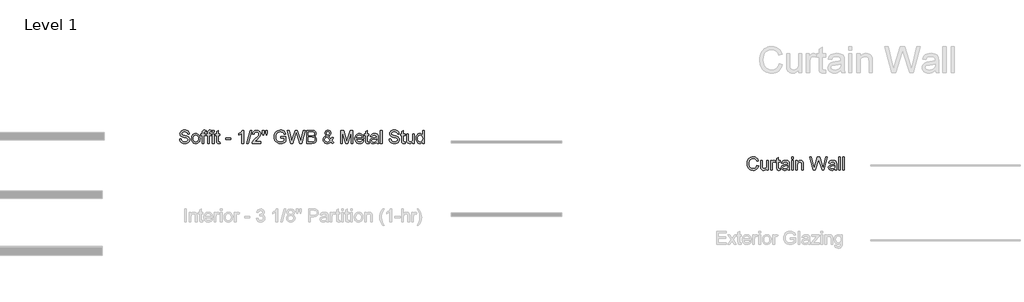
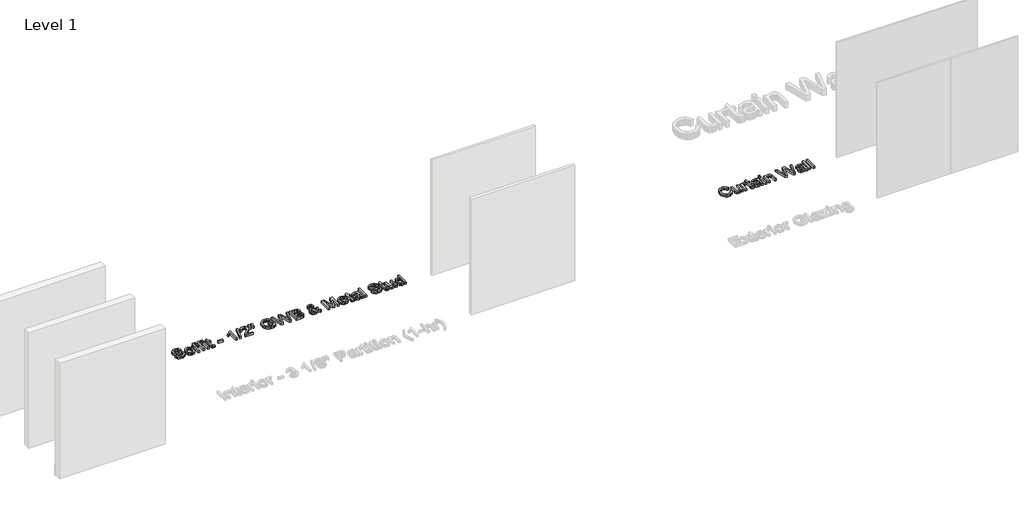
# One storey, part 40 of 42: 2 proxies.
"""IFC4 building model written with IfcOpenShell, lengths in millimetres."""

from ifc_helpers import new_model, si_unit, origin, origin_with_axes, place, context, project, spatial, polyline, outline, extrude, element, save

model = new_model("IFC4")

# Units and contexts
model_context = context("Model", 3, world=origin())
ifc_project = project(units=[si_unit("LENGTHUNIT", "METRE", prefix="MILLI")], contexts=[model_context])

# Site, building, storey
site = spatial("IfcSite", under=ifc_project)
building = spatial("IfcBuilding", under=site)
storey = spatial("IfcBuildingStorey", under=building, Name="Level 1", Elevation=0.0)

# Proxies
placement = place(None, origin())
element("IfcBuildingElementProxy", 1, Name="8\" Arial", ObjectType="8\" Arial", at=placement, inside=storey, context=model_context, shape_type="SweptSolid", body=[
    extrude(outline(polyline([(5120.6223042, 17413.5110871), (5158.693191, 17413.5110871), (5163.0616765, 17392.3843474), (5170.9621291, 17375.4030217), (5183.2868351, 17361.9257791), (5200.928081, 17351.3112887), (5222.4916692, 17344.423953), (5246.5834022, 17342.1281744), (5267.7937937, 17343.866274), (5286.3645046, 17349.0805727), (5301.4125431, 17357.3342219), (5312.0549174, 17368.1903732), (5318.3845741, 17380.654499), (5320.4944597, 17393.7320717), (5318.9143692, 17406.4750369), (5314.1740976, 17417.4891973), (5304.5448402, 17426.8860885), (5288.2977918, 17434.7772465), (5232.8644987, 17449.3140792), (5196.4759436, 17458.934042), (5173.1928451, 17468.0892724), (5154.2410536, 17480.8973002), (5140.8102842, 17496.4193658), (5132.8075905, 17514.3208619), (5130.1400259, 17534.267181), (5133.4396267, 17556.5650466), (5143.338429, 17577.3571788), (5159.5761827, 17594.9798354), (5181.8926376, 17607.7692739), (5208.6798191, 17615.548896), (5238.3297529, 17618.1421034), (5270.4520636, 17615.4280656), (5298.5590855, 17607.2859521), (5321.6469963, 17593.8830667), (5338.7119739, 17575.386713), (5349.5123573, 17552.9494277), (5353.8064856, 17527.7237473), (5315.7355989, 17527.7237473), (5308.746022, 17550.4398722), (5294.1720107, 17566.8356349), (5271.4001179, 17576.7623212), (5239.8168969, 17580.0712166), (5207.4901039, 17576.7994998), (5185.3130688, 17566.9843493), (5172.4864517, 17552.5404631), (5168.2109127, 17535.382539), (5171.2409686, 17520.7527598), (5180.3311364, 17508.9857328), (5201.8203674, 17498.4641889), (5242.4937562, 17487.7195734), (5284.468396, 17477.5140476), (5309.86138, 17468.6097728), (5331.564388, 17454.7979228), (5346.7053729, 17437.7515345), (5355.6003531, 17417.656501), (5358.5653465, 17394.6987153), (5355.1542099, 17371.2297238), (5344.9208001, 17349.1549299), (5328.2833765, 17330.1566651), (5305.6601982, 17315.9172611), (5278.4547574, 17307.022281), (5248.0705462, 17304.0572876), (5210.7711154, 17307.2546473), (5180.0708862, 17316.8467262), (5155.6166618, 17332.8707029), (5137.0552456, 17355.3637561), (5125.1395042, 17382.7643846), (5120.6223042, 17413.5110871)])), origin_with_axes(), (0.0, 0.0, 1.0), 50.8),
    extrude(outline(polyline([(5401.3950941, 17420.6493783), (5403.4538591, 17449.6161553), (5409.630154, 17474.5769381), (5419.923979, 17495.5317268), (5434.335334, 17512.4805212), (5448.8442828, 17523.3134359), (5464.8589649, 17531.0512321), (5482.3793803, 17535.6939098), (5501.405529, 17537.241469), (5522.4091145, 17535.3569787), (5541.4004083, 17529.7035078), (5558.3794104, 17520.2810563), (5573.3461207, 17507.0896241), (5585.5616146, 17490.5753546), (5594.2869673, 17471.1843909), (5599.522179, 17448.9167329), (5601.2672495, 17423.7723808), (5598.1814257, 17385.3111187), (5588.9239542, 17356.0329709), (5573.7643799, 17334.1068914), (5552.9722477, 17317.701834), (5528.2763624, 17307.4684242), (5501.405529, 17304.0572876), (5480.09522, 17305.934807), (5460.9273279, 17311.5673649), (5443.9018526, 17320.9549615), (5429.0187941, 17334.0975967), (5416.9334253, 17350.772199), (5408.3010191, 17370.7556967), (5403.1215753, 17394.0480898), (5401.3950941, 17420.6493783)]), holes=[polyline([(5439.4659808, 17420.7237355), (5443.871645, 17386.2684677), (5457.0886374, 17361.7212968), (5476.9791886, 17347.026455), (5501.405529, 17342.1281744), (5525.7203336, 17347.0543389), (5545.5737062, 17361.8328326), (5558.7906986, 17386.7053162), (5563.1963628, 17421.9134507), (5558.7628147, 17455.3648964), (5545.4621704, 17479.5774599), (5525.5809139, 17494.2723017), (5501.405529, 17499.1705823), (5476.9791886, 17494.290891), (5457.0886374, 17479.6518171), (5443.871645, 17455.1604141), (5439.4659808, 17420.7237355)])]), origin_with_axes(), (0.0, 0.0, 1.0), 50.8),
    extrude(outline(polyline([(5653.6147188, 17308.8161485), (5653.6147188, 17494.4117214), (5620.3026929, 17494.4117214), (5620.3026929, 17532.4826082), (5653.6147188, 17532.4826082), (5653.6147188, 17555.01284), (5657.6300077, 17586.7633647), (5665.2887993, 17599.4226781), (5677.1115943, 17609.4423109), (5693.6560714, 17615.9671553), (5715.4799098, 17618.1421034), (5750.2047225, 17613.9781002), (5744.6279325, 17578.2866438), (5722.6925583, 17580.0712166), (5708.2207881, 17578.4911261), (5698.7123611, 17573.7508546), (5693.4422945, 17564.6978654), (5691.6856056, 17550.179622), (5691.6856056, 17532.4826082), (5734.5153532, 17532.4826082), (5734.5153532, 17494.4117214), (5691.6856056, 17494.4117214), (5691.6856056, 17308.8161485), (5653.6147188, 17308.8161485)])), origin_with_axes(), (0.0, 0.0, 1.0), 50.8),
    extrude(outline(polyline([(5777.3451008, 17308.8161485), (5777.3451008, 17494.4117214), (5744.0330749, 17494.4117214), (5744.0330749, 17532.4826082), (5777.3451008, 17532.4826082), (5777.3451008, 17555.01284), (5781.3603896, 17586.7633647), (5789.0191813, 17599.4226781), (5800.8419762, 17609.4423109), (5817.3864534, 17615.9671553), (5839.2102918, 17618.1421034), (5873.9351045, 17613.9781002), (5868.3583145, 17578.2866438), (5846.4229403, 17580.0712166), (5831.9511701, 17578.4911261), (5822.442743, 17573.7508546), (5817.1726764, 17564.6978654), (5815.4159876, 17550.179622), (5815.4159876, 17532.4826082), (5858.2457352, 17532.4826082), (5858.2457352, 17494.4117214), (5815.4159876, 17494.4117214), (5815.4159876, 17308.8161485), (5777.3451008, 17308.8161485)])), origin_with_axes(), (0.0, 0.0, 1.0), 50.8),
    extrude(outline(polyline([(5891.5577611, 17575.3123558), (5891.5577611, 17613.3832425), (5929.6286478, 17613.3832425), (5929.6286478, 17575.3123558), (5891.5577611, 17575.3123558)])), origin_with_axes(), (0.0, 0.0, 1.0), 50.8),
    extrude(outline(polyline([(5891.5577611, 17308.8161485), (5891.5577611, 17532.4826082), (5929.6286478, 17532.4826082), (5929.6286478, 17308.8161485), (5891.5577611, 17308.8161485)])), origin_with_axes(), (0.0, 0.0, 1.0), 50.8),
    extrude(outline(polyline([(6067.6356123, 17340.5666732), (6072.3944732, 17307.7007905), (6043.9156653, 17304.0572876), (6025.6423832, 17305.6373781), (6012.0164262, 17310.3776497), (6002.3871687, 17317.6832447), (5996.1039853, 17326.9593055), (5992.6463754, 17342.8903357), (5991.4938388, 17370.1608391), (5991.4938388, 17494.4117214), (5962.9406738, 17494.4117214), (5962.9406738, 17532.4826082), (5991.4938388, 17532.4826082), (5991.4938388, 17586.8377219), (6029.5647256, 17609.2192393), (6029.5647256, 17532.4826082), (6067.6356123, 17532.4826082), (6067.6356123, 17494.4117214), (6029.5647256, 17494.4117214), (6029.5647256, 17371.2761971), (6031.57237, 17351.6458961), (6038.0786251, 17344.6934978), (6051.0539566, 17342.1281744), (6067.6356123, 17340.5666732)])), origin_with_axes(), (0.0, 0.0, 1.0), 50.8),
    extrude(outline(polyline([(6205.6425768, 17399.2345045), (6205.6425768, 17437.3053913), (6324.614098, 17437.3053913), (6324.614098, 17399.2345045), (6205.6425768, 17399.2345045)])), origin_with_axes(), (0.0, 0.0, 1.0), 50.8),
    extrude(outline(polyline([(6619.6634703, 17308.8161485), (6581.5925836, 17308.8161485), (6581.5925836, 17546.1643331), (6545.5293412, 17520.4739203), (6505.4508101, 17501.2525839), (6505.4508101, 17537.241469), (6535.3516994, 17553.5071067), (6561.2558892, 17572.8585682), (6581.6762354, 17593.4369235), (6595.1255941, 17613.3832425), (6619.6634703, 17613.3832425), (6619.6634703, 17308.8161485)])), origin_with_axes(), (0.0, 0.0, 1.0), 50.8),
    extrude(outline(polyline([(6691.046383, 17308.8161485), (6776.7058782, 17613.3832425), (6811.0589049, 17613.3832425), (6725.3994097, 17308.8161485), (6691.046383, 17308.8161485)])), origin_with_axes(), (0.0, 0.0, 1.0), 50.8),
    extrude(outline(polyline([(7024.1666421, 17346.8870352), (7024.1666421, 17308.8161485), (6824.2944867, 17308.8161485), (6828.3841327, 17335.0642403), (6837.7717293, 17355.5775331), (6851.5092221, 17375.4773789), (6871.381184, 17396.3066898), (6899.1721878, 17419.6083775), (6940.2545412, 17456.0991738), (6964.9039532, 17483.0350697), (6977.2286592, 17504.8960867), (6981.3368945, 17526.1622461), (6977.4610255, 17545.2255735), (6965.8334182, 17561.0729519), (6947.9598061, 17571.7525048), (6925.3459224, 17575.3123558), (6901.5980914, 17571.8361567), (6883.148211, 17561.4075593), (6871.2417643, 17544.8444928), (6867.1242343, 17522.9648865), (6829.0533475, 17527.7237473), (6832.327388, 17547.377285), (6838.282935, 17564.549151), (6846.9199886, 17579.2393455), (6858.2385488, 17591.4478683), (6871.9783653, 17601.0445946), (6887.8791879, 17607.899399), (6926.1638516, 17613.3832425), (6946.5679322, 17611.8589199), (6964.7273548, 17607.2859521), (6980.6421194, 17599.664339), (6994.3122261, 17588.9940807), (7005.2915315, 17576.0652224), (7013.1338925, 17561.6678095), (7017.8393091, 17545.8018418), (7019.4077813, 17528.4673193), (7017.716155, 17510.2590998), (7012.641276, 17492.3668984), (7003.6347601, 17474.1679735), (6990.1482228, 17455.0395837), (6968.6496972, 17432.2026284), (6935.6072161, 17402.8780074), (6891.8108249, 17366.257086), (6874.6343115, 17346.8870352), (7024.1666421, 17346.8870352)])), origin_with_axes(), (0.0, 0.0, 1.0), 50.8),
    extrude(outline(polyline([(7147.4508809, 17503.9294431), (7138.3793024, 17562.7459889), (7138.3793024, 17613.3832425), (7176.4501892, 17613.3832425), (7176.4501892, 17562.7459889), (7167.5273251, 17503.9294431), (7147.4508809, 17503.9294431)])), origin_with_axes(), (0.0, 0.0, 1.0), 50.8),
    extrude(outline(polyline([(7071.532179, 17503.9294431), (7062.2375289, 17562.7459889), (7062.2375289, 17613.3832425), (7100.3084157, 17613.3832425), (7100.3084157, 17562.7459889), (7091.9804092, 17503.9294431), (7071.532179, 17503.9294431)])), origin_with_axes(), (0.0, 0.0, 1.0), 50.8),
    extrude(outline(polyline([(7490.5350049, 17427.7876696), (7490.5350049, 17465.8585564), (7614.2653869, 17465.8585564), (7614.2653869, 17352.0176821), (7584.1971939, 17331.1047194), (7553.1809465, 17316.1031541), (7521.2910021, 17307.0687543), (7488.6017177, 17304.0572876), (7445.8928006, 17308.8440324), (7407.2921188, 17323.2042668), (7375.225576, 17346.6360797), (7352.1190758, 17378.6375599), (7338.1492168, 17417.0244648), (7333.4925971, 17459.6125515), (7338.1306275, 17502.5073617), (7352.0447186, 17542.4092945), (7374.6586023, 17575.8793294), (7389.0118657, 17588.9127525), (7405.3960101, 17599.478446), (7442.8348607, 17613.476189), (7485.5530725, 17618.1421034), (7516.9132219, 17615.4373602), (7545.1131903, 17607.3231307), (7568.8610212, 17594.3849778), (7586.8647584, 17577.2084644), (7600.183992, 17554.9663667), (7609.8783121, 17526.8314609), (7574.7817133, 17516.9419532), (7566.9463233, 17537.0091028), (7557.419307, 17552.1500878), (7544.8157615, 17563.5639181), (7527.7507839, 17572.4496036), (7507.4047948, 17578.1658134), (7484.9582149, 17580.0712166), (7458.6822391, 17578.017099), (7436.2170698, 17571.854746), (7417.646359, 17562.3556136), (7403.0537583, 17550.2911578), (7383.4606359, 17520.9572421), (7374.5377718, 17492.218184), (7371.5634838, 17461.1740527), (7375.1419241, 17424.7669083), (7385.877245, 17394.8102511), (7403.4441336, 17371.517858), (7427.5172773, 17355.1035059), (7455.6893618, 17345.3720073), (7485.5530725, 17342.1281744), (7511.9219948, 17344.5726674), (7537.6402916, 17351.9061463), (7559.9753357, 17362.0094309), (7576.1945001, 17372.7633411), (7576.1945001, 17427.7876696), (7490.5350049, 17427.7876696)])), origin_with_axes(), (0.0, 0.0, 1.0), 50.8),
    extrude(outline(polyline([(7730.634406, 17308.8161485), (7647.5774128, 17613.3832425), (7686.8380148, 17613.3832425), (7735.0214808, 17413.2136583), (7749.892921, 17351.4228245), (7765.8053619, 17406.075367), (7826.1834089, 17613.3832425), (7882.7692386, 17613.3832425), (7926.639987, 17463.1073399), (7945.4337695, 17407.3394394), (7959.2827982, 17351.4228245), (7973.7080951, 17411.4290854), (8022.3377043, 17613.3832425), (8061.5983063, 17613.3832425), (7978.4669559, 17308.8161485), (7937.7935672, 17308.8161485), (7864.7747961, 17543.7849027), (7854.5878596, 17576.5764282), (7843.1368507, 17537.0927546), (7776.587156, 17308.8161485), (7730.634406, 17308.8161485)])), origin_with_axes(), (0.0, 0.0, 1.0), 50.8),
    extrude(outline(polyline([(8099.6691931, 17308.8161485), (8099.6691931, 17613.3832425), (8215.8894978, 17613.3832425), (8247.8537994, 17611.1432319), (8272.8099349, 17604.4231999), (8291.9383248, 17593.0558428), (8306.4193896, 17576.873857), (8315.5374414, 17557.8384136), (8318.5767919, 17537.9106838), (8316.0207632, 17519.5723392), (8308.3526768, 17502.3307633), (8295.5167651, 17487.2455462), (8277.45726, 17475.376278), (8299.0301428, 17464.1111621), (8314.9704677, 17446.9718274), (8324.8135021, 17425.0922211), (8328.0945136, 17399.6062905), (8325.854503, 17378.3680151), (8319.1344709, 17358.6726515), (8309.1055435, 17341.9236921), (8296.9388465, 17329.5246289), (8282.0395224, 17320.5459969), (8263.8127136, 17314.0583311), (8214.9972114, 17308.8161485), (8099.6691931, 17308.8161485)]), holes=[polyline([(8137.7400798, 17489.6528606), (8207.2640625, 17489.6528606), (8247.8630941, 17492.9245774), (8262.0746141, 17498.56643), (8272.2894345, 17507.0152669), (8278.4517875, 17518.1409631), (8280.5059052, 17531.8133934), (8278.5912073, 17545.0861537), (8272.8471135, 17556.6486984), (8263.5338741, 17565.6738036), (8250.9117393, 17571.3342456), (8201.9847012, 17575.3123558), (8137.7400798, 17575.3123558), (8137.7400798, 17489.6528606)]), polyline([(8137.7400798, 17346.8870352), (8215.8151406, 17346.8870352), (8244.0708768, 17348.3741793), (8267.9767169, 17356.6650071), (8283.8148006, 17373.5812703), (8288.4714203, 17385.5341903), (8290.0236269, 17399.2345045), (8288.2018755, 17415.1469455), (8282.7366212, 17428.8286704), (8273.1910156, 17439.5268127), (8259.12821, 17446.4885056), (8239.2097748, 17450.3086068), (8212.0972805, 17451.5819738), (8137.7400798, 17451.5819738), (8137.7400798, 17346.8870352)])]), origin_with_axes(), (0.0, 0.0, 1.0), 50.8),
    extrude(outline(polyline([(8669.3197076, 17346.440892), (8649.9682462, 17327.8980651), (8628.9437477, 17314.6531887), (8606.2090335, 17306.7062629), (8581.7269252, 17304.0572876), (8559.5127115, 17306.0184588), (8539.7151068, 17311.9019723), (8522.3341112, 17321.7078282), (8507.3697245, 17335.4360263), (8490.6951223, 17362.5206367), (8485.1369215, 17392.6167137), (8489.6076482, 17419.2923594), (8503.0198283, 17443.2539673), (8525.3176938, 17464.4829481), (8556.445477, 17482.9607125), (8529.8627777, 17521.4777425), (8523.2078083, 17550.0309076), (8528.4499909, 17575.7399097), (8544.1765389, 17597.8425876), (8567.840718, 17613.0672244), (8596.8957942, 17618.1421034), (8624.5380835, 17613.290296), (8646.6407614, 17598.734874), (8661.1404156, 17577.3757681), (8665.9736336, 17552.1129092), (8662.3951933, 17530.9025177), (8651.6598725, 17511.290806), (8633.7676711, 17493.2777741), (8608.7185891, 17476.8634221), (8663.8172748, 17408.2317258), (8673.2048714, 17427.8434375), (8680.2502161, 17450.3922586), (8718.3211029, 17442.1386093), (8706.6098438, 17406.8747069), (8691.4037962, 17379.4554891), (8713.0417417, 17354.2112195), (8737.3565463, 17333.3540247), (8708.8033812, 17304.0572876), (8689.3775625, 17321.8286586), (8669.3197076, 17346.440892)]), holes=[polyline([(8589.4600741, 17500.8807979), (8609.3692146, 17513.5122274), (8620.7644556, 17524.4892091), (8626.118174, 17535.1687621), (8627.9027469, 17546.9079051), (8625.5512004, 17560.2085494), (8618.496561, 17570.8137451), (8607.9099545, 17577.7568488), (8594.9625069, 17580.0712166), (8581.7362199, 17577.7754381), (8570.9079525, 17570.8881023), (8563.6860094, 17560.6918712), (8561.278695, 17548.4694063), (8564.5504119, 17534.5274312), (8574.4399195, 17519.0239549), (8589.4600741, 17500.8807979)]), polyline([(8643.8151878, 17373.8786991), (8575.8527064, 17458.7202651), (8549.8927487, 17442.1571986), (8534.026781, 17426.821026), (8525.9125514, 17412.1726575), (8523.2078083, 17397.6730033), (8526.907079, 17379.7157393), (8538.0048912, 17361.0892606), (8555.887798, 17346.8684459), (8579.9423524, 17342.1281744), (8597.165339, 17344.3403011), (8614.9274153, 17350.9766813), (8631.165169, 17361.1264392), (8643.8151878, 17373.8786991)])]), origin_with_axes(), (0.0, 0.0, 1.0), 50.8),
    extrude(outline(polyline([(8899.157815, 17308.8161485), (8899.157815, 17613.3832425), (8964.6665088, 17613.3832425), (9026.977843, 17398.7140041), (9039.5442099, 17353.8766121), (9053.1515777, 17402.4318642), (9114.421911, 17613.3832425), (9179.9306048, 17613.3832425), (9179.9306048, 17308.8161485), (9141.8597181, 17308.8161485), (9141.8597181, 17575.3123558), (9065.3461586, 17308.8161485), (9013.7422613, 17308.8161485), (8937.2287018, 17575.3123558), (8937.2287018, 17308.8161485), (8899.157815, 17308.8161485)])), origin_with_axes(), (0.0, 0.0, 1.0), 50.8),
    extrude(outline(polyline([(9398.3920605, 17375.4402003), (9435.7193753, 17370.6813395), (9422.2700166, 17342.5557283), (9400.8086695, 17321.5312298), (9371.8186559, 17308.4257732), (9335.7832975, 17304.0572876), (9312.1609443, 17305.9417779), (9291.1132092, 17311.5952489), (9272.6400921, 17321.0177004), (9256.7415932, 17334.2091325), (9243.956802, 17350.8024066), (9234.8248083, 17370.4303839), (9229.345612, 17393.0930645), (9227.5192133, 17418.7904483), (9229.3642013, 17445.3592056), (9234.8991655, 17468.7770765), (9244.1241057, 17489.044061), (9257.039022, 17506.1601591), (9272.895695, 17519.7582322), (9290.9459055, 17529.4711416), (9311.1896534, 17535.2988872), (9333.6269387, 17537.241469), (9355.341565, 17535.3035345), (9374.9788369, 17529.4897309), (9392.5387546, 17519.8000581), (9408.021318, 17506.2345163), (9420.6597185, 17489.1555968), (9429.6871474, 17468.9257909), (9435.1036047, 17445.5450986), (9436.9090905, 17419.0135199), (9436.6860189, 17408.7522262), (9265.5901001, 17408.7522262), (9272.180007, 17380.2548291), (9287.4882957, 17359.3046878), (9309.5816789, 17346.4223027), (9336.5268695, 17342.1281744), (9356.7892067, 17344.1172295), (9373.8541843, 17350.0843949), (9387.7218022, 17360.4014565), (9398.3920605, 17375.4402003)]), holes=[polyline([(9265.5901001, 17446.823113), (9398.8382037, 17446.823113), (9393.6889676, 17466.9367358), (9383.5949776, 17481.3248541), (9361.3993532, 17494.7091502), (9333.4782243, 17499.1705823), (9307.8156954, 17495.6107313), (9286.5960093, 17484.9311783), (9271.8453996, 17468.28446), (9265.5901001, 17446.823113)])]), origin_with_axes(), (0.0, 0.0, 1.0), 50.8),
    extrude(outline(polyline([(9555.8806116, 17340.5666732), (9560.6394724, 17307.7007905), (9532.1606646, 17304.0572876), (9513.8873825, 17305.6373781), (9500.2614255, 17310.3776497), (9490.632168, 17317.6832447), (9484.3489845, 17326.9593055), (9480.8913747, 17342.8903357), (9479.7388381, 17370.1608391), (9479.7388381, 17494.4117214), (9451.185673, 17494.4117214), (9451.185673, 17532.4826082), (9479.7388381, 17532.4826082), (9479.7388381, 17586.8377219), (9517.8097248, 17609.2192393), (9517.8097248, 17532.4826082), (9555.8806116, 17532.4826082), (9555.8806116, 17494.4117214), (9517.8097248, 17494.4117214), (9517.8097248, 17371.2761971), (9519.8173693, 17351.6458961), (9526.3236243, 17344.6934978), (9539.2989558, 17342.1281744), (9555.8806116, 17340.5666732)])), origin_with_axes(), (0.0, 0.0, 1.0), 50.8),
    extrude(outline(polyline([(9736.7173237, 17337.3693135), (9718.5276935, 17321.7728907), (9699.7989735, 17311.5673649), (9680.10361, 17305.934807), (9659.014049, 17304.0572876), (9627.1984617, 17308.5744876), (9603.7294702, 17322.1260874), (9589.2577001, 17342.7044427), (9584.4337767, 17368.301909), (9586.2555281, 17384.0842249), (9591.7207823, 17398.4165753), (9600.15103, 17410.6855134), (9610.8677615, 17420.2775923), (9637.524818, 17432.769602), (9670.4650579, 17438.4951065), (9709.3910524, 17444.5180398), (9736.4942521, 17451.5819738), (9736.7173237, 17460.0586947), (9734.0962324, 17477.0493151), (9726.2329584, 17488.1657166), (9708.6474804, 17496.4193658), (9684.1467828, 17499.1705823), (9661.4678366, 17497.3395362), (9645.6297528, 17491.846398), (9634.8293694, 17481.6873455), (9627.2635243, 17465.8585564), (9589.1926375, 17470.6174172), (9595.8011337, 17491.4374334), (9605.6627575, 17507.7960176), (9619.6976791, 17520.3066166), (9638.826069, 17529.5826774), (9662.2207032, 17535.3267711), (9689.054358, 17537.241469), (9714.7912441, 17535.5498427), (9735.1930011, 17530.4749638), (9750.575647, 17522.844056), (9761.2551999, 17513.4843434), (9768.3377233, 17501.912504), (9772.9292804, 17487.6452162), (9774.7882105, 17454.3331902), (9774.7882105, 17406.9676534), (9776.7214977, 17340.8269234), (9784.3059321, 17308.8161485), (9746.2350454, 17308.8161485), (9740.1377549, 17322.0517302), (9736.7173237, 17337.3693135)]), holes=[polyline([(9736.7173237, 17413.5110871), (9675.2982759, 17401.8370066), (9642.543929, 17395.6653589), (9627.7096675, 17385.6271368), (9622.5046634, 17370.9787683), (9625.3395317, 17359.6578845), (9633.8441365, 17350.3818237), (9647.8325849, 17344.1915867), (9667.1189838, 17342.1281744), (9687.567214, 17344.4053637), (9705.6360138, 17351.2369315), (9720.2843823, 17361.3030375), (9730.4713188, 17373.2838415), (9734.9885188, 17385.6271368), (9736.4942521, 17402.729293), (9736.7173237, 17413.5110871)])]), origin_with_axes(), (0.0, 0.0, 1.0), 50.8),
    extrude(outline(polyline([(9827.1356797, 17308.8161485), (9827.1356797, 17613.3832425), (9865.2065665, 17613.3832425), (9865.2065665, 17308.8161485), (9827.1356797, 17308.8161485)])), origin_with_axes(), (0.0, 0.0, 1.0), 50.8),
    extrude(outline(polyline([(10031.7666961, 17413.5110871), (10069.8375828, 17413.5110871), (10074.2060684, 17392.3843474), (10082.1065209, 17375.4030217), (10094.431227, 17361.9257791), (10112.0724728, 17351.3112887), (10133.636061, 17344.423953), (10157.7277941, 17342.1281744), (10178.9381856, 17343.866274), (10197.5088964, 17349.0805727), (10212.5569349, 17357.3342219), (10223.1993093, 17368.1903732), (10229.528966, 17380.654499), (10231.6388516, 17393.7320717), (10230.058761, 17406.4750369), (10225.3184895, 17417.4891973), (10215.689232, 17426.8860885), (10199.4421837, 17434.7772465), (10144.0088905, 17449.3140792), (10107.6203354, 17458.934042), (10084.337237, 17468.0892724), (10065.3854454, 17480.8973002), (10051.9546761, 17496.4193658), (10043.9519823, 17514.3208619), (10041.2844178, 17534.267181), (10044.5840185, 17556.5650466), (10054.4828209, 17577.3571788), (10070.7205746, 17594.9798354), (10093.0370294, 17607.7692739), (10119.824211, 17615.548896), (10149.4741448, 17618.1421034), (10181.5964555, 17615.4280656), (10209.7034773, 17607.2859521), (10232.7913882, 17593.8830667), (10249.8563657, 17575.386713), (10260.6567491, 17552.9494277), (10264.9508775, 17527.7237473), (10226.8799907, 17527.7237473), (10219.8904138, 17550.4398722), (10205.3164025, 17566.8356349), (10182.5445098, 17576.7623212), (10150.9612888, 17580.0712166), (10118.6344958, 17576.7994998), (10096.4574607, 17566.9843493), (10083.6308436, 17552.5404631), (10079.3553045, 17535.382539), (10082.3853604, 17520.7527598), (10091.4755282, 17508.9857328), (10112.9647592, 17498.4641889), (10153.638148, 17487.7195734), (10195.6127878, 17477.5140476), (10221.0057719, 17468.6097728), (10242.7087798, 17454.7979228), (10257.8497648, 17437.7515345), (10266.7447449, 17417.656501), (10269.7097383, 17394.6987153), (10266.2986017, 17371.2297238), (10256.065192, 17349.1549299), (10239.4277683, 17330.1566651), (10216.80459, 17315.9172611), (10189.5991492, 17307.022281), (10159.2149381, 17304.0572876), (10121.9155073, 17307.2546473), (10091.215278, 17316.8467262), (10066.7610537, 17332.8707029), (10048.1996374, 17355.3637561), (10036.283896, 17382.7643846), (10031.7666961, 17413.5110871)])), origin_with_axes(), (0.0, 0.0, 1.0), 50.8),
    extrude(outline(polyline([(10402.957842, 17340.5666732), (10407.7167028, 17307.7007905), (10379.2378949, 17304.0572876), (10360.9646129, 17305.6373781), (10347.3386558, 17310.3776497), (10337.7093984, 17317.6832447), (10331.4262149, 17326.9593055), (10327.9686051, 17342.8903357), (10326.8160685, 17370.1608391), (10326.8160685, 17494.4117214), (10298.2629034, 17494.4117214), (10298.2629034, 17532.4826082), (10326.8160685, 17532.4826082), (10326.8160685, 17586.8377219), (10364.8869552, 17609.2192393), (10364.8869552, 17532.4826082), (10402.957842, 17532.4826082), (10402.957842, 17494.4117214), (10364.8869552, 17494.4117214), (10364.8869552, 17371.2761971), (10366.8945996, 17351.6458961), (10373.4008547, 17344.6934978), (10386.3761862, 17342.1281744), (10402.957842, 17340.5666732)])), origin_with_axes(), (0.0, 0.0, 1.0), 50.8),
    extrude(outline(polyline([(10583.7945541, 17308.8161485), (10583.7945541, 17347.2588212), (10570.0198826, 17328.3581503), (10553.9773166, 17314.857671), (10535.6668559, 17306.7573835), (10515.0885006, 17304.0572876), (10496.5456737, 17305.9533963), (10479.2855085, 17311.6417221), (10464.8044436, 17320.1928002), (10454.5989179, 17330.6771655), (10447.7301714, 17343.4108361), (10443.2594447, 17358.7098301), (10441.0287287, 17394.1038577), (10441.0287287, 17532.4826082), (10479.0996155, 17532.4826082), (10479.0996155, 17412.0239431), (10481.4046887, 17373.2094843), (10486.9535948, 17360.2620367), (10496.4620218, 17350.4190023), (10509.2979336, 17344.2008814), (10524.8292939, 17342.1281744), (10541.2529406, 17344.2473546), (10556.6169972, 17350.6048953), (10569.2856053, 17360.6152334), (10577.6229064, 17373.6928061), (10582.2516422, 17391.6035968), (10583.7945541, 17416.1135891), (10583.7945541, 17532.4826082), (10621.8654408, 17532.4826082), (10621.8654408, 17308.8161485), (10583.7945541, 17308.8161485)])), origin_with_axes(), (0.0, 0.0, 1.0), 50.8),
    extrude(outline(polyline([(10812.2198746, 17308.8161485), (10812.2198746, 17344.7306764), (10800.8292809, 17326.9360688), (10787.0313729, 17314.2256348), (10770.8261505, 17306.5993744), (10752.2136137, 17304.0572876), (10727.6013802, 17307.7379691), (10705.0711484, 17318.7800134), (10685.9985264, 17336.4119646), (10671.7591225, 17359.8623668), (10662.8920263, 17388.1831656), (10659.9363276, 17420.4263067), (10662.6596601, 17452.2697779), (10670.8296575, 17481.0274253), (10684.4370252, 17505.0633904), (10703.4724686, 17522.7418149), (10726.4953169, 17533.6165555), (10752.0648993, 17537.241469), (10770.691378, 17534.6482617), (10787.161498, 17526.8686395), (10801.1220624, 17514.9436035), (10812.2198746, 17499.9141543), (10812.2198746, 17613.3832425), (10850.2907614, 17613.3832425), (10850.2907614, 17308.8161485), (10812.2198746, 17308.8161485)]), holes=[polyline([(10698.0072143, 17420.5750211), (10702.3013427, 17386.1383426), (10715.1837277, 17361.6469396), (10733.903153, 17347.0078657), (10755.7084021, 17342.1281744), (10777.5043565, 17346.7847941), (10795.7497547, 17360.7546532), (10808.1023446, 17384.2980018), (10812.2198746, 17417.6750903), (10808.0279874, 17454.1658865), (10795.4523259, 17479.4659241), (10776.7421952, 17494.2444177), (10754.1469009, 17499.1705823), (10732.1185802, 17494.4396054), (10714.0683697, 17480.2466747), (10702.0225032, 17455.8668075), (10698.0072143, 17420.5750211)])]), origin_with_axes(), (0.0, 0.0, 1.0), 50.8),
])
element("IfcBuildingElementProxy", 2, Name="8\" Arial", ObjectType="8\" Arial", at=placement, inside=storey, context=model_context, shape_type="SweptSolid", body=[
    extrude(outline(polyline([(18644.690255, 16788.4879383), (18682.7611417, 16778.6727878), (18675.2278278, 16754.9969903), (18665.1942531, 16734.3094229), (18652.6604174, 16716.6100855), (18637.6263209, 16701.898978), (18620.4312182, 16690.3341097), (18601.4143642, 16682.0734894), (18580.5757587, 16677.1171172), (18557.9154018, 16675.4649932), (18513.7565192, 16680.4655149), (18495.0858908, 16686.7161671), (18478.6878044, 16695.4670802), (18451.8076764, 16719.9491885), (18432.214554, 16753.3913395), (18420.2523393, 16792.7077094), (18416.2649344, 16834.8124743), (18420.7728397, 16879.2223124), (18434.2965556, 16917.5720387), (18456.1296886, 16948.6440539), (18485.5658455, 16971.220759), (18520.4765512, 16984.9675465), (18558.733331, 16989.549809), (18580.5083725, 16988.0673123), (18600.4756045, 16983.6198222), (18618.6350271, 16976.2073387), (18634.9866403, 16965.8298619), (18649.2608992, 16952.7615839), (18661.1882589, 16937.2766969), (18678.0022809, 16899.0570957), (18639.9313941, 16889.9855172), (18626.732991, 16917.748637), (18608.7013698, 16936.7933751), (18585.613459, 16947.8075354), (18557.2461869, 16951.4789222), (18524.5476079, 16947.4078655), (18497.6860692, 16935.1946952), (18477.3029015, 16916.1220733), (18464.0394359, 16891.4726612), (18456.7617249, 16863.6073003), (18454.3358212, 16834.8868315), (18457.2078681, 16799.7158756), (18465.8240087, 16769.3037805), (18480.5095558, 16744.8123775), (18501.5898222, 16727.4034979), (18526.8619758, 16717.0027844), (18554.1231845, 16713.53588), (18585.9015932, 16718.2575622), (18612.3820513, 16732.4226089), (18632.3748436, 16755.8823057), (18644.690255, 16788.4879383)])), origin_with_axes(), (0.0, 0.0, 1.0), 50.8),
    extrude(outline(polyline([(18873.1155755, 16680.223854), (18873.1155755, 16718.6665268), (18859.3409041, 16699.7658558), (18843.298338, 16686.2653766), (18824.9878774, 16678.165089), (18804.4095221, 16675.4649932), (18785.8666952, 16677.3611018), (18768.6065299, 16683.0494277), (18754.1254651, 16691.6005057), (18743.9199393, 16702.084871), (18737.0511929, 16714.8185417), (18732.5804662, 16730.1175357), (18730.3497502, 16765.5115632), (18730.3497502, 16903.8903137), (18768.4206369, 16903.8903137), (18768.4206369, 16783.4316486), (18770.7257102, 16744.6171898), (18776.2746163, 16731.6697423), (18785.7830433, 16721.8267078), (18798.6189551, 16715.6085869), (18814.1503154, 16713.53588), (18830.5739621, 16715.6550602), (18845.9380187, 16722.0126008), (18858.6066267, 16732.022939), (18866.9439279, 16745.1005116), (18871.5726636, 16763.0113024), (18873.1155755, 16787.5212946), (18873.1155755, 16903.8903137), (18911.1864623, 16903.8903137), (18911.1864623, 16680.223854), (18873.1155755, 16680.223854)])), origin_with_axes(), (0.0, 0.0, 1.0), 50.8),
    extrude(outline(polyline([(18963.5339316, 16680.223854), (18963.5339316, 16903.8903137), (18996.8459575, 16903.8903137), (18996.8459575, 16870.8013594), (19009.1520742, 16889.9855172), (19020.4915473, 16901.2878117), (19031.868199, 16906.8088339), (19044.2858515, 16908.6491746), (19063.2469377, 16905.7120652), (19082.5054527, 16896.9007369), (19069.7903714, 16862.7707818), (19056.4060752, 16868.6264113), (19043.0217791, 16870.5782878), (19031.6544221, 16868.7007685), (19021.4953695, 16863.0682106), (19013.2881935, 16854.1081679), (19007.776466, 16842.2481944), (19003.1477302, 16820.982035), (19001.6048183, 16797.7825883), (19001.6048183, 16680.223854), (18963.5339316, 16680.223854)])), origin_with_axes(), (0.0, 0.0, 1.0), 50.8),
    extrude(outline(polyline([(19187.2003913, 16711.9743787), (19191.9592521, 16679.108496), (19163.4804443, 16675.4649932), (19145.2071622, 16677.0450837), (19131.5812052, 16681.7853553), (19121.9519477, 16689.0909502), (19115.6687642, 16698.367011), (19112.2111544, 16714.2980413), (19111.0586178, 16741.5685446), (19111.0586178, 16865.819427), (19082.5054527, 16865.819427), (19082.5054527, 16903.8903137), (19111.0586178, 16903.8903137), (19111.0586178, 16958.2454275), (19149.1295045, 16980.6269449), (19149.1295045, 16903.8903137), (19187.2003913, 16903.8903137), (19187.2003913, 16865.819427), (19149.1295045, 16865.819427), (19149.1295045, 16742.6839026), (19151.1371489, 16723.0536016), (19157.643404, 16716.1012034), (19170.6187355, 16713.53588), (19187.2003913, 16711.9743787)])), origin_with_axes(), (0.0, 0.0, 1.0), 50.8),
    extrude(outline(polyline([(19368.0371034, 16708.7770191), (19349.8474732, 16693.1805963), (19331.1187532, 16682.9750705), (19311.4233897, 16677.3425125), (19290.3338287, 16675.4649932), (19258.5182414, 16679.9821931), (19235.0492499, 16693.533793), (19220.5774797, 16714.1121483), (19215.7535564, 16739.7096146), (19217.5753078, 16755.4919304), (19223.040562, 16769.8242809), (19231.4708096, 16782.093219), (19242.1875412, 16791.6852979), (19268.8445977, 16804.1773076), (19301.7848376, 16809.9028121), (19340.7108321, 16815.9257453), (19367.8140318, 16822.9896794), (19368.0371034, 16831.4664003), (19365.4160121, 16848.4570206), (19357.5527381, 16859.5734221), (19339.9672601, 16867.8270714), (19315.4665625, 16870.5782878), (19292.7876163, 16868.7472418), (19276.9495325, 16863.2541036), (19266.1491491, 16853.095051), (19258.583304, 16837.2662619), (19220.5124172, 16842.0251228), (19227.1209134, 16862.845139), (19236.9825371, 16879.2037231), (19251.0174588, 16891.7143221), (19270.1458487, 16900.9903829), (19293.5404829, 16906.7344767), (19320.3741377, 16908.6491746), (19346.1110238, 16906.9575483), (19366.5127808, 16901.8826693), (19381.8954267, 16894.2517616), (19392.5749796, 16884.892049), (19399.657503, 16873.3202096), (19404.2490601, 16859.0529217), (19406.1079901, 16825.7408958), (19406.1079901, 16778.375359), (19408.0412774, 16712.2346289), (19415.6257118, 16680.223854), (19377.5548251, 16680.223854), (19371.4575346, 16693.4594358), (19368.0371034, 16708.7770191)]), holes=[polyline([(19368.0371034, 16784.9187926), (19306.6180556, 16773.2447121), (19273.8637087, 16767.0730645), (19259.0294472, 16757.0348424), (19253.8244431, 16742.3864738), (19256.6593114, 16731.06559), (19265.1639162, 16721.7895292), (19279.1523646, 16715.5992923), (19298.4387635, 16713.53588), (19318.8869937, 16715.8130692), (19336.9557935, 16722.644637), (19351.604162, 16732.7107431), (19361.7910985, 16744.691547), (19366.3082985, 16757.0348424), (19367.8140318, 16774.1369985), (19368.0371034, 16784.9187926)])]), origin_with_axes(), (0.0, 0.0, 1.0), 50.8),
    extrude(outline(polyline([(19458.4554594, 16680.223854), (19458.4554594, 16903.8903137), (19496.5263462, 16903.8903137), (19496.5263462, 16680.223854), (19458.4554594, 16680.223854)])), origin_with_axes(), (0.0, 0.0, 1.0), 50.8),
    extrude(outline(polyline([(19458.4554594, 16946.7200613), (19458.4554594, 16984.7909481), (19496.5263462, 16984.7909481), (19496.5263462, 16946.7200613), (19458.4554594, 16946.7200613)])), origin_with_axes(), (0.0, 0.0, 1.0), 50.8),
    extrude(outline(polyline([(19553.6326763, 16680.223854), (19553.6326763, 16903.8903137), (19591.7035631, 16903.8903137), (19591.7035631, 16872.6602894), (19604.9298502, 16888.4054267), (19620.8144072, 16899.6519533), (19639.3572341, 16906.3998693), (19660.5583309, 16908.6491746), (19679.3242295, 16906.8367178), (19696.5100375, 16901.3993475), (19710.8423879, 16893.0155731), (19721.0479137, 16882.3639041), (19732.461744, 16854.3684181), (19734.4693884, 16817.5616037), (19734.4693884, 16680.223854), (19696.3985017, 16680.223854), (19696.3985017, 16812.4309569), (19692.0114268, 16846.1147688), (19685.9420203, 16856.1436962), (19676.5079505, 16863.9233184), (19664.4156107, 16868.9145455), (19650.3713944, 16870.5782878), (19628.0735289, 16866.8418385), (19609.0659695, 16855.6324905), (19601.4699167, 16846.4819075), (19596.0441647, 16833.9759558), (19591.7035631, 16798.8979464), (19591.7035631, 16680.223854), (19553.6326763, 16680.223854)])), origin_with_axes(), (0.0, 0.0, 1.0), 50.8),
    extrude(outline(polyline([(19965.0510678, 16680.223854), (19881.9940746, 16984.7909481), (19921.2546766, 16984.7909481), (19969.4381426, 16784.6213638), (19984.3095828, 16722.83053), (20000.2220237, 16777.4830726), (20060.6000707, 16984.7909481), (20117.1859004, 16984.7909481), (20161.0566489, 16834.5150455), (20179.8504313, 16778.747145), (20193.69946, 16722.83053), (20208.1247569, 16782.836791), (20256.7543662, 16984.7909481), (20296.0149681, 16984.7909481), (20212.8836177, 16680.223854), (20172.210229, 16680.223854), (20099.1914579, 16915.1926083), (20089.0045214, 16947.9841338), (20077.5535125, 16908.5004602), (20011.0038178, 16680.223854), (19965.0510678, 16680.223854)])), origin_with_axes(), (0.0, 0.0, 1.0), 50.8),
    extrude(outline(polyline([(20472.0928194, 16708.7770191), (20453.9031892, 16693.1805963), (20435.1744692, 16682.9750705), (20415.4791057, 16677.3425125), (20394.3895447, 16675.4649932), (20362.5739574, 16679.9821931), (20339.1049659, 16693.533793), (20324.6331957, 16714.1121483), (20319.8092723, 16739.7096146), (20321.6310238, 16755.4919304), (20327.096278, 16769.8242809), (20335.5265256, 16782.093219), (20346.2432572, 16791.6852979), (20372.9003136, 16804.1773076), (20405.8405536, 16809.9028121), (20444.7665481, 16815.9257453), (20471.8697478, 16822.9896794), (20472.0928194, 16831.4664003), (20469.4717281, 16848.4570206), (20461.6084541, 16859.5734221), (20444.0229761, 16867.8270714), (20419.5222785, 16870.5782878), (20396.8433323, 16868.7472418), (20381.0052485, 16863.2541036), (20370.2048651, 16853.095051), (20362.63902, 16837.2662619), (20324.5681332, 16842.0251228), (20331.1766294, 16862.845139), (20341.0382531, 16879.2037231), (20355.0731748, 16891.7143221), (20374.2015647, 16900.9903829), (20397.5961989, 16906.7344767), (20424.4298537, 16908.6491746), (20450.1667398, 16906.9575483), (20470.5684968, 16901.8826693), (20485.9511427, 16894.2517616), (20496.6306956, 16884.892049), (20503.713219, 16873.3202096), (20508.3047761, 16859.0529217), (20510.1637061, 16825.7408958), (20510.1637061, 16778.375359), (20512.0969934, 16712.2346289), (20519.6814278, 16680.223854), (20481.6105411, 16680.223854), (20475.5132506, 16693.4594358), (20472.0928194, 16708.7770191)]), holes=[polyline([(20472.0928194, 16784.9187926), (20410.6737716, 16773.2447121), (20377.9194247, 16767.0730645), (20363.0851632, 16757.0348424), (20357.8801591, 16742.3864738), (20360.7150274, 16731.06559), (20369.2196322, 16721.7895292), (20383.2080806, 16715.5992923), (20402.4944795, 16713.53588), (20422.9427097, 16715.8130692), (20441.0115095, 16722.644637), (20455.659878, 16732.7107431), (20465.8468145, 16744.691547), (20470.3640145, 16757.0348424), (20471.8697478, 16774.1369985), (20472.0928194, 16784.9187926)])]), origin_with_axes(), (0.0, 0.0, 1.0), 50.8),
    extrude(outline(polyline([(20562.5111754, 16680.223854), (20562.5111754, 16984.7909481), (20600.5820622, 16984.7909481), (20600.5820622, 16680.223854), (20562.5111754, 16680.223854)])), origin_with_axes(), (0.0, 0.0, 1.0), 50.8),
    extrude(outline(polyline([(20657.6883923, 16680.223854), (20657.6883923, 16984.7909481), (20695.7592791, 16984.7909481), (20695.7592791, 16680.223854), (20657.6883923, 16680.223854)])), origin_with_axes(), (0.0, 0.0, 1.0), 50.8),
])

save(model, "model.ifc")

# Revit data of these elements
# Elements 1, 2 (IfcBuildingElementProxy, "8\" Arial")
#   Phase Created = New Construction
